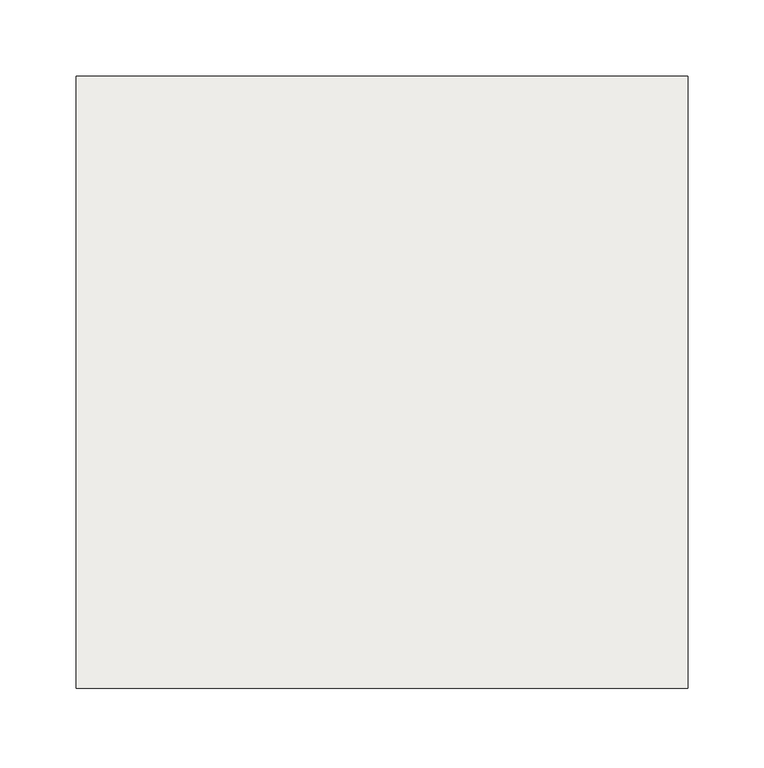
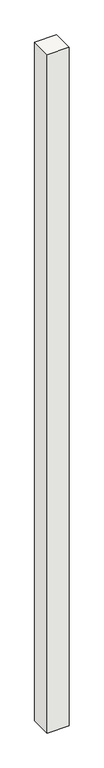
"""IFC4 building model written with IfcOpenShell, lengths in millimetres: slab geometry, NLRS_17_SFO_TLB_funderingspaal geheid beton prefab-AV-MMBPC_gen_rsf : heipaal beton prefab_gen__bxh 400x400."""

from ifc_helpers import new_model, si_unit, frame, origin, place, context, project, spatial, polyline, outline, extrude, source, transform, mapped, element, save


def slab_443494b9(model_context):
    return source(origin(), model_context, "Body", "SweptSolid", [
        extrude(outline(polyline([(200.0, -200.0), (-200.0, -200.0), (-200.0, 200.0), (200.0, 200.0), (200.0, -200.0)])), frame((0.0, 0.0, -20000.0), z_axis=(0.0, 0.0, 1.0), x_axis=(1.0, 0.0, 0.0)), (0.0, 0.0, 1.0), 13220.0),
    ])


if __name__ == "__main__":
    model = new_model("IFC4")
    model_context = context("Model", 3, world=origin())
    ifc_project = project(units=[si_unit("LENGTHUNIT", "METRE", prefix="MILLI")], contexts=[model_context])
    site = spatial("IfcSite", under=ifc_project)
    building = spatial("IfcBuilding", under=site)
    placement = place(None, origin())
    slab_shape = slab_443494b9(model_context)
    element("IfcSlab", 1, ObjectType="NLRS_17_SFO_TLB_funderingspaal geheid beton prefab-AV-MMBPC_gen_rsf : heipaal beton prefab_gen__bxh 400x400", at=placement, inside=building, context=model_context, shape_type="MappedRepresentation", body=[
        mapped(slab_shape, transform((0.0, 0.0, 0.0), x_axis=(1.0, 0.0, 0.0), y_axis=(0.0, 1.0, 0.0), z_axis=(0.0, 0.0, 1.0))),
    ])
    save(model, "model.ifc")

# Revit data of these elements
# Type "NLRS_17_SFO_TLB_funderingspaal geheid beton prefab-AV-MMBPC_gen_rsf : heipaal beton prefab_gen__bxh 400x400"
#   Export Type to IFC As = "IfcPile"
#   Type IfcGUID = "10$Kfo5uPCAOPJEOo5LE_W"
#   Type Comments = "prefab heipaal 400x400"
#   Model = " "
#   Manufacturer = " "
#   Description = "prefab heipaal 400x400"
#   Assembly Code = "17.21"
#   Width = 400 mm
#   Slanted Angle [instance default] = 0.00°
#   NLRS_S_draagvermogen_trek [instance default] = 0.00 kN
#   NLRS_S_draagvermogen_druk [instance default] = 0.00 kN
#   NLRS_C_lengte [instance default] = 1660 mm
#   NLRS_C_hoogte = 400 mm
#   NLRS_C_breedte = 400 mm
#   Height [instance default] = 1660 mm
#   Length [instance default] = 1660 mm
#   Angle [instance default] = 0.00°
#   Slanted [instance default] = 0
#   Structural Material = NLRS_f2_beton prefab_gen_rsf
#   Keynote = ""
# Element 1 (IfcSlab, "NLRS_17_SFO_TLB_funderingspaal geheid beton prefab-AV-MMBPC_gen_rsf : heipaal beton prefab_gen__bxh 400x400")
#   NLRS_C_lengte = 13220 mm
#   Height = 13220 mm
#   Length = 13220 mm
#   Materials on its faces: "NLRS_f2_beton prefab_gen_rsf"
# Materials
#   "NLRS_f2_beton prefab_gen_rsf": class "F - Niet gebakken kunststeen", colour RGB 129 133 118, transparency 0, Keynote = "f2", Manufacturer = "Revit Standards Foundation", URL = "www.revitstandards.org", Description = "beton prefab", Cost = 0
